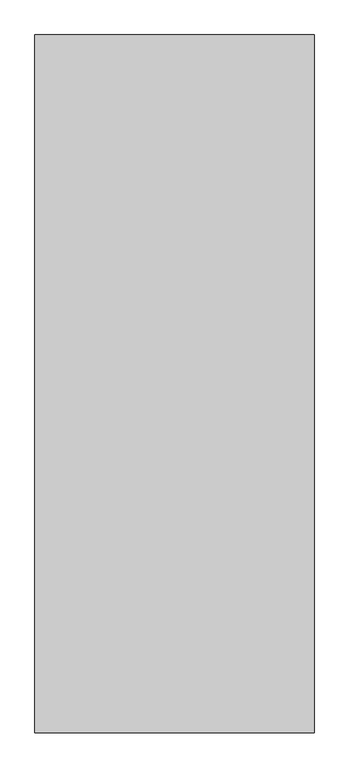
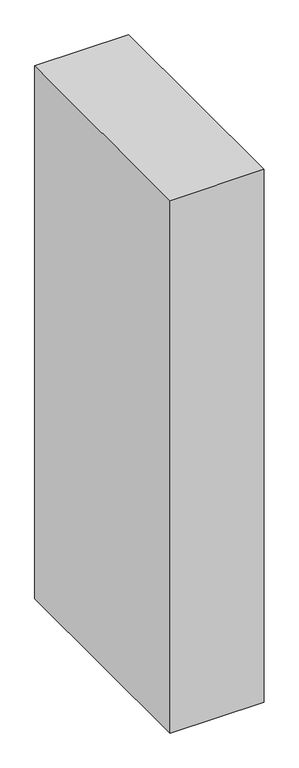
"""IFC4 building model written with IfcOpenShell, lengths in millimetres: proxy geometry, Space Planning Box_hec : Space Planning Box_hec."""

from ifc_helpers import new_model, si_unit, origin, origin_with_axes, place, context, project, spatial, polyline, outline, extrude, source, transform, mapped, element, save


def generic_models_71e2440f(model_context):
    return source(origin(), model_context, "Body", "SweptSolid", [
        extrude(outline(polyline([(500.0, 1250.0), (500.0, -1250.0), (-500.0, -1250.0), (-500.0, 1250.0), (500.0, 1250.0)])), origin_with_axes(), (0.0, 0.0, 1.0), 6000.0),
    ])


if __name__ == "__main__":
    model = new_model("IFC4")
    model_context = context("Model", 3, world=origin())
    ifc_project = project(units=[si_unit("LENGTHUNIT", "METRE", prefix="MILLI")], contexts=[model_context])
    site = spatial("IfcSite", under=ifc_project)
    building = spatial("IfcBuilding", under=site)
    placement = place(None, origin())
    generic_models_shape = generic_models_71e2440f(model_context)
    element("IfcBuildingElementProxy", 1, Name="Space Planning Box_hec : Space Planning Box_hec", ObjectType="Space Planning Box_hec : Space Planning Box_hec", at=placement, inside=building, context=model_context, shape_type="MappedRepresentation", body=[
        mapped(generic_models_shape, transform((0.0, 0.0, 0.0), x_axis=(1.0, 0.0, 0.0), y_axis=(0.0, 1.0, 0.0), z_axis=(0.0, 0.0, 1.0))),
    ])
    save(model, "model.ifc")

# Revit data of these elements
# Type "Space Planning Box_hec : Space Planning Box_hec"
#   Type Comments = "..."
#   Room Name [instance default] = "?"
#   Interior Finish [instance default] = ""
#   Exterior Finish [instance default] = ""
#   Department [instance default] = ""
#   Assembly Code = "..."
#   Width [instance default] = 1524 mm
#   Program Area [instance default] = 0 m²
#   Length [instance default] = 1524 mm
#   Height [instance default] = 1524 mm
#   Area [instance default] = 2.32258 m²
#   Fill Color [instance default] = Cyan
#   Default Elevation = 0
# Element 1 (IfcBuildingElementProxy, "Space Planning Box_hec : Space Planning Box_hec")
#   Room Name = "Pipe Shaft"
#   Interior Finish = "NA"
#   Exterior Finish = "EF1"
#   Department = "HV"
#   Width = 1000 mm
#   Program Area = 2.5 m²
#   Length = 2500 mm
#   Height = 6000 mm
#   Area = 2.5 m²
#   Fill Color = Pink
#   Materials on its faces: "Pink"
# Materials
#   "Cyan": class "Generic", colour RGB 0 255 255, transparency 0.2, Cost = 0
#   "Pink": class "Generic", colour RGB 255 105 180, transparency 0.2, Cost = 0
